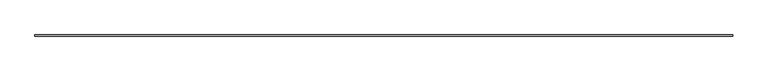
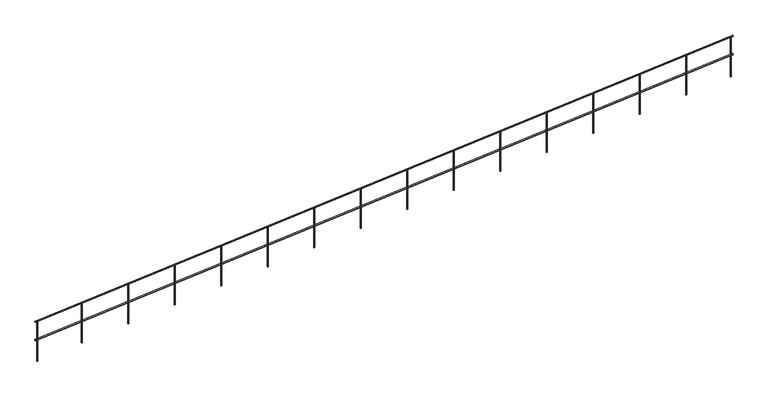
"""IFC4 building model written with IfcOpenShell, lengths in millimetres: railing geometry."""

from ifc_helpers import new_model, si_unit, frame, origin, place, context, project, spatial, ellipse_curve, source, transform, mapped, element, save
from ifc_brep_helpers import plane_surface, cylinder_surface, advanced_brep


def railing_ef706f2a(model_context):
    return source(origin(), model_context, "Body", "AdvancedBrep", [
        advanced_brep(
        [(42716.32048, 67987.0208589, -615.0519932), (42716.32048, 68017.0208589, -615.0519932), (60716.32048, 67987.0208589, 884.9480068), (60716.32048, 68017.0208589, 884.9480068)],
        [
            (0, 1, ellipse_curve(frame((42716.32048, 68002.0208589, -615.0519932), z_axis=(-1.0, 0.0, 0.0), x_axis=(0.0, 0.0, -0.9999999999999999)), 15.0519932, 15.0)),
            (1, 0, ellipse_curve(frame((42716.32048, 68002.0208589, -615.0519932), z_axis=(-1.0, 0.0, 0.0), x_axis=(0.0, 0.0, -0.9999999999999999)), 15.0519932, 15.0)),
            (2, 3, ellipse_curve(frame((60716.32048, 68002.0208589, 884.9480068), z_axis=(1.0, 0.0, 0.0), x_axis=(0.0, 0.0, -0.9999999999999999)), 15.0519932, 15.0)),
            (3, 2, ellipse_curve(frame((60716.32048, 68002.0208589, 884.9480068), z_axis=(1.0, 0.0, 0.0), x_axis=(0.0, 0.0, -0.9999999999999999)), 15.0519932, 15.0)),
            (0, 2),
            (3, 1),
        ],
        [
            plane_surface(frame((42716.32048, 68002.0208589, -600.0), z_axis=(-1.0, 0.0, 0.0), x_axis=(0.0, 1.0, 0.0))),
            plane_surface(frame((60716.32048, 68002.0208589, 900.0), z_axis=(1.0, 0.0, 0.0), x_axis=(0.0, 1.0, 0.0))),
            cylinder_surface(frame((42717.5661622, 68002.0208589, -614.9481864), z_axis=(-0.9965457582448797, 0.0, -0.08304547985373997), x_axis=(0.0, 1.0, 0.0)), 15.0),
        ],
        [
            (0, [[1, 2]]),
            (1, [[3, 4]]),
            (2, [[-1, 5, -4, 6]]),
            (2, [[-2, -6, -3, -5]]),
        ],
    ),
        advanced_brep(
        [(42716.32048, 67987.0208589, -115.0519932), (42716.32048, 68017.0208589, -115.0519932), (60716.32048, 67987.0208589, 1384.9480068), (60716.32048, 68017.0208589, 1384.9480068)],
        [
            (0, 1, ellipse_curve(frame((42716.32048, 68002.0208589, -115.0519932), z_axis=(-1.0, 0.0, 0.0), x_axis=(0.0, 0.0, -0.9999999999999999)), 15.0519932, 15.0)),
            (1, 0, ellipse_curve(frame((42716.32048, 68002.0208589, -115.0519932), z_axis=(-1.0, 0.0, 0.0), x_axis=(0.0, 0.0, -0.9999999999999999)), 15.0519932, 15.0)),
            (2, 3, ellipse_curve(frame((60716.32048, 68002.0208589, 1384.9480068), z_axis=(1.0, 0.0, 0.0), x_axis=(0.0, 0.0, -0.9999999999999999)), 15.0519932, 15.0)),
            (3, 2, ellipse_curve(frame((60716.32048, 68002.0208589, 1384.9480068), z_axis=(1.0, 0.0, 0.0), x_axis=(0.0, 0.0, -0.9999999999999999)), 15.0519932, 15.0)),
            (0, 2),
            (3, 1),
        ],
        [
            plane_surface(frame((42716.32048, 68002.0208589, -100.0), z_axis=(-1.0, 0.0, 0.0), x_axis=(0.0, 1.0, 0.0))),
            plane_surface(frame((60716.32048, 68002.0208589, 1400.0), z_axis=(1.0, 0.0, 0.0), x_axis=(0.0, 1.0, 0.0))),
            cylinder_surface(frame((42717.5661622, 68002.0208589, -114.9481864), z_axis=(-0.9965457582448797, 0.0, -0.08304547985373997), x_axis=(0.0, 1.0, 0.0)), 15.0),
        ],
        [
            (0, [[1, 2]]),
            (1, [[3, 4]]),
            (2, [[-1, 5, -4, 6]]),
            (2, [[-2, -6, -3, -5]]),
        ],
    ),
        advanced_brep(
        [(59516.32048, 68017.0208589, 1269.8960136), (59516.32048, 67987.0208589, 1269.8960136), (59516.32048, 67987.0208589, 200.0), (59516.32048, 68017.0208589, 200.0)],
        [
            (0, 1, ellipse_curve(frame((59516.32048, 68002.0208589, 1269.8960136), z_axis=(0.083045479853741, 0.0, -0.9965457582448796), x_axis=(0.9965457582448797, 0.0, 0.08304547985374044)), 15.0519932, 15.0)),
            (1, 2),
            (2, 3, ellipse_curve(frame((59516.32048, 68002.0208589, 200.0), z_axis=(-0.08304547985373996, 0.0, 0.9965457582448797), x_axis=(0.9965457582448798, 0.0, 0.08304547985373881)), 15.0519932, 15.0)),
            (3, 0),
            (3, 2, ellipse_curve(frame((59516.32048, 68002.0208589, 200.0), z_axis=(-0.08304547985373996, 0.0, 0.9965457582448797), x_axis=(0.9965457582448798, 0.0, 0.08304547985373881)), 15.0519932, 15.0)),
            (1, 0, ellipse_curve(frame((59516.32048, 68002.0208589, 1269.8960136), z_axis=(0.083045479853741, 0.0, -0.9965457582448796), x_axis=(0.9965457582448797, 0.0, 0.08304547985374044)), 15.0519932, 15.0)),
        ],
        [
            cylinder_surface(frame((59516.32048, 68002.0208589, 100.0), z_axis=(0.0, 0.0, 1.0), x_axis=(0.0, -1.0, 0.0)), 15.0),
            plane_surface(frame((59541.32048, 67977.0208589, 1271.9793469), z_axis=(-0.083045479853741, 0.0, 0.9965457582448796), x_axis=(0.0, 1.0, 0.0))),
            plane_surface(frame((59491.32048, 67977.0208589, 197.9166667), z_axis=(0.08304547985373996, 0.0, -0.9965457582448797), x_axis=(0.0, 1.0, 0.0))),
        ],
        [
            (0, [[1, 2, 3, 4]]),
            (0, [[5, -2, 6, -4]]),
            (1, [[-6, -1]]),
            (2, [[-5, -3]]),
        ],
    ),
        advanced_brep(
        [(58316.32048, 68017.0208589, 1169.8960136), (58316.32048, 67987.0208589, 1169.8960136), (58316.32048, 67987.0208589, 100.0), (58316.32048, 68017.0208589, 100.0)],
        [
            (0, 1, ellipse_curve(frame((58316.32048, 68002.0208589, 1169.8960136), z_axis=(0.083045479853741, 0.0, -0.9965457582448796), x_axis=(0.9965457582448797, 0.0, 0.08304547985374044)), 15.0519932, 15.0)),
            (1, 2),
            (2, 3, ellipse_curve(frame((58316.32048, 68002.0208589, 100.0), z_axis=(-0.08304547985373996, 0.0, 0.9965457582448797), x_axis=(0.9965457582448798, 0.0, 0.08304547985373881)), 15.0519932, 15.0)),
            (3, 0),
            (3, 2, ellipse_curve(frame((58316.32048, 68002.0208589, 100.0), z_axis=(-0.08304547985373996, 0.0, 0.9965457582448797), x_axis=(0.9965457582448798, 0.0, 0.08304547985373881)), 15.0519932, 15.0)),
            (1, 0, ellipse_curve(frame((58316.32048, 68002.0208589, 1169.8960136), z_axis=(0.083045479853741, 0.0, -0.9965457582448796), x_axis=(0.9965457582448797, 0.0, 0.08304547985374044)), 15.0519932, 15.0)),
        ],
        [
            cylinder_surface(frame((58316.32048, 68002.0208589, 0.0), z_axis=(0.0, 0.0, 1.0), x_axis=(0.0, -1.0, 0.0)), 15.0),
            plane_surface(frame((58341.32048, 67977.0208589, 1171.9793469), z_axis=(-0.083045479853741, 0.0, 0.9965457582448796), x_axis=(0.0, 1.0, 0.0))),
            plane_surface(frame((58291.32048, 67977.0208589, 97.9166667), z_axis=(0.08304547985373996, 0.0, -0.9965457582448797), x_axis=(0.0, 1.0, 0.0))),
        ],
        [
            (0, [[1, 2, 3, 4]]),
            (0, [[5, -2, 6, -4]]),
            (1, [[-6, -1]]),
            (2, [[-5, -3]]),
        ],
    ),
        advanced_brep(
        [(57116.32048, 68017.0208589, 1069.8960136), (57116.32048, 67987.0208589, 1069.8960136), (57116.32048, 67987.0208589, 0.0), (57116.32048, 68017.0208589, 0.0)],
        [
            (0, 1, ellipse_curve(frame((57116.32048, 68002.0208589, 1069.8960136), z_axis=(0.083045479853741, 0.0, -0.9965457582448796), x_axis=(0.9965457582448797, 0.0, 0.08304547985374044)), 15.0519932, 15.0)),
            (1, 2),
            (2, 3, ellipse_curve(frame((57116.32048, 68002.0208589, 0.0), z_axis=(-0.08304547985373996, 0.0, 0.9965457582448797), x_axis=(0.9965457582448798, 0.0, 0.08304547985373881)), 15.0519932, 15.0)),
            (3, 0),
            (3, 2, ellipse_curve(frame((57116.32048, 68002.0208589, 0.0), z_axis=(-0.08304547985373996, 0.0, 0.9965457582448797), x_axis=(0.9965457582448798, 0.0, 0.08304547985373881)), 15.0519932, 15.0)),
            (1, 0, ellipse_curve(frame((57116.32048, 68002.0208589, 1069.8960136), z_axis=(0.083045479853741, 0.0, -0.9965457582448796), x_axis=(0.9965457582448797, 0.0, 0.08304547985374044)), 15.0519932, 15.0)),
        ],
        [
            cylinder_surface(frame((57116.32048, 68002.0208589, -100.0), z_axis=(0.0, 0.0, 1.0), x_axis=(0.0, -1.0, 0.0)), 15.0),
            plane_surface(frame((57141.32048, 67977.0208589, 1071.9793469), z_axis=(-0.083045479853741, 0.0, 0.9965457582448796), x_axis=(0.0, 1.0, 0.0))),
            plane_surface(frame((57091.32048, 67977.0208589, -2.0833333), z_axis=(0.08304547985373996, 0.0, -0.9965457582448797), x_axis=(0.0, 1.0, 0.0))),
        ],
        [
            (0, [[1, 2, 3, 4]]),
            (0, [[5, -2, 6, -4]]),
            (1, [[-6, -1]]),
            (2, [[-5, -3]]),
        ],
    ),
        advanced_brep(
        [(55916.32048, 68017.0208589, 969.8960136), (55916.32048, 67987.0208589, 969.8960136), (55916.32048, 67987.0208589, -100.0), (55916.32048, 68017.0208589, -100.0)],
        [
            (0, 1, ellipse_curve(frame((55916.32048, 68002.0208589, 969.8960136), z_axis=(0.083045479853741, 0.0, -0.9965457582448796), x_axis=(0.9965457582448797, 0.0, 0.08304547985374044)), 15.0519932, 15.0)),
            (1, 2),
            (2, 3, ellipse_curve(frame((55916.32048, 68002.0208589, -100.0), z_axis=(-0.08304547985373996, 0.0, 0.9965457582448797), x_axis=(0.9965457582448798, 0.0, 0.08304547985373881)), 15.0519932, 15.0)),
            (3, 0),
            (3, 2, ellipse_curve(frame((55916.32048, 68002.0208589, -100.0), z_axis=(-0.08304547985373996, 0.0, 0.9965457582448797), x_axis=(0.9965457582448798, 0.0, 0.08304547985373881)), 15.0519932, 15.0)),
            (1, 0, ellipse_curve(frame((55916.32048, 68002.0208589, 969.8960136), z_axis=(0.083045479853741, 0.0, -0.9965457582448796), x_axis=(0.9965457582448797, 0.0, 0.08304547985374044)), 15.0519932, 15.0)),
        ],
        [
            cylinder_surface(frame((55916.32048, 68002.0208589, -200.0), z_axis=(0.0, 0.0, 1.0), x_axis=(0.0, -1.0, 0.0)), 15.0),
            plane_surface(frame((55941.32048, 67977.0208589, 971.9793469), z_axis=(-0.083045479853741, 0.0, 0.9965457582448796), x_axis=(0.0, 1.0, 0.0))),
            plane_surface(frame((55891.32048, 67977.0208589, -102.0833333), z_axis=(0.08304547985373996, 0.0, -0.9965457582448797), x_axis=(0.0, 1.0, 0.0))),
        ],
        [
            (0, [[1, 2, 3, 4]]),
            (0, [[5, -2, 6, -4]]),
            (1, [[-6, -1]]),
            (2, [[-5, -3]]),
        ],
    ),
        advanced_brep(
        [(54716.32048, 68017.0208589, 869.8960136), (54716.32048, 67987.0208589, 869.8960136), (54716.32048, 67987.0208589, -200.0), (54716.32048, 68017.0208589, -200.0)],
        [
            (0, 1, ellipse_curve(frame((54716.32048, 68002.0208589, 869.8960136), z_axis=(0.083045479853741, 0.0, -0.9965457582448796), x_axis=(0.9965457582448797, 0.0, 0.08304547985374044)), 15.0519932, 15.0)),
            (1, 2),
            (2, 3, ellipse_curve(frame((54716.32048, 68002.0208589, -200.0), z_axis=(-0.08304547985373996, 0.0, 0.9965457582448797), x_axis=(0.9965457582448798, 0.0, 0.08304547985373881)), 15.0519932, 15.0)),
            (3, 0),
            (3, 2, ellipse_curve(frame((54716.32048, 68002.0208589, -200.0), z_axis=(-0.08304547985373996, 0.0, 0.9965457582448797), x_axis=(0.9965457582448798, 0.0, 0.08304547985373881)), 15.0519932, 15.0)),
            (1, 0, ellipse_curve(frame((54716.32048, 68002.0208589, 869.8960136), z_axis=(0.083045479853741, 0.0, -0.9965457582448796), x_axis=(0.9965457582448797, 0.0, 0.08304547985374044)), 15.0519932, 15.0)),
        ],
        [
            cylinder_surface(frame((54716.32048, 68002.0208589, -300.0), z_axis=(0.0, 0.0, 1.0), x_axis=(0.0, -1.0, 0.0)), 15.0),
            plane_surface(frame((54741.32048, 67977.0208589, 871.9793469), z_axis=(-0.083045479853741, 0.0, 0.9965457582448796), x_axis=(0.0, 1.0, 0.0))),
            plane_surface(frame((54691.32048, 67977.0208589, -202.0833333), z_axis=(0.08304547985373996, 0.0, -0.9965457582448797), x_axis=(0.0, 1.0, 0.0))),
        ],
        [
            (0, [[1, 2, 3, 4]]),
            (0, [[5, -2, 6, -4]]),
            (1, [[-6, -1]]),
            (2, [[-5, -3]]),
        ],
    ),
        advanced_brep(
        [(53516.32048, 68017.0208589, 769.8960136), (53516.32048, 67987.0208589, 769.8960136), (53516.32048, 67987.0208589, -300.0), (53516.32048, 68017.0208589, -300.0)],
        [
            (0, 1, ellipse_curve(frame((53516.32048, 68002.0208589, 769.8960136), z_axis=(0.083045479853741, 0.0, -0.9965457582448796), x_axis=(0.9965457582448797, 0.0, 0.08304547985374044)), 15.0519932, 15.0)),
            (1, 2),
            (2, 3, ellipse_curve(frame((53516.32048, 68002.0208589, -300.0), z_axis=(-0.08304547985373996, 0.0, 0.9965457582448797), x_axis=(0.9965457582448798, 0.0, 0.08304547985373881)), 15.0519932, 15.0)),
            (3, 0),
            (3, 2, ellipse_curve(frame((53516.32048, 68002.0208589, -300.0), z_axis=(-0.08304547985373996, 0.0, 0.9965457582448797), x_axis=(0.9965457582448798, 0.0, 0.08304547985373881)), 15.0519932, 15.0)),
            (1, 0, ellipse_curve(frame((53516.32048, 68002.0208589, 769.8960136), z_axis=(0.083045479853741, 0.0, -0.9965457582448796), x_axis=(0.9965457582448797, 0.0, 0.08304547985374044)), 15.0519932, 15.0)),
        ],
        [
            cylinder_surface(frame((53516.32048, 68002.0208589, -400.0), z_axis=(0.0, 0.0, 1.0), x_axis=(0.0, -1.0, 0.0)), 15.0),
            plane_surface(frame((53541.32048, 67977.0208589, 771.9793469), z_axis=(-0.083045479853741, 0.0, 0.9965457582448796), x_axis=(0.0, 1.0, 0.0))),
            plane_surface(frame((53491.32048, 67977.0208589, -302.0833333), z_axis=(0.08304547985373996, 0.0, -0.9965457582448797), x_axis=(0.0, 1.0, 0.0))),
        ],
        [
            (0, [[1, 2, 3, 4]]),
            (0, [[5, -2, 6, -4]]),
            (1, [[-6, -1]]),
            (2, [[-5, -3]]),
        ],
    ),
        advanced_brep(
        [(52316.32048, 68017.0208589, 669.8960136), (52316.32048, 67987.0208589, 669.8960136), (52316.32048, 67987.0208589, -400.0), (52316.32048, 68017.0208589, -400.0)],
        [
            (0, 1, ellipse_curve(frame((52316.32048, 68002.0208589, 669.8960136), z_axis=(0.083045479853741, 0.0, -0.9965457582448796), x_axis=(0.9965457582448797, 0.0, 0.08304547985374044)), 15.0519932, 15.0)),
            (1, 2),
            (2, 3, ellipse_curve(frame((52316.32048, 68002.0208589, -400.0), z_axis=(-0.08304547985373996, 0.0, 0.9965457582448797), x_axis=(0.9965457582448798, 0.0, 0.08304547985373881)), 15.0519932, 15.0)),
            (3, 0),
            (3, 2, ellipse_curve(frame((52316.32048, 68002.0208589, -400.0), z_axis=(-0.08304547985373996, 0.0, 0.9965457582448797), x_axis=(0.9965457582448798, 0.0, 0.08304547985373881)), 15.0519932, 15.0)),
            (1, 0, ellipse_curve(frame((52316.32048, 68002.0208589, 669.8960136), z_axis=(0.083045479853741, 0.0, -0.9965457582448796), x_axis=(0.9965457582448797, 0.0, 0.08304547985374044)), 15.0519932, 15.0)),
        ],
        [
            cylinder_surface(frame((52316.32048, 68002.0208589, -500.0), z_axis=(0.0, 0.0, 1.0), x_axis=(0.0, -1.0, 0.0)), 15.0),
            plane_surface(frame((52341.32048, 67977.0208589, 671.9793469), z_axis=(-0.083045479853741, 0.0, 0.9965457582448796), x_axis=(0.0, 1.0, 0.0))),
            plane_surface(frame((52291.32048, 67977.0208589, -402.0833333), z_axis=(0.08304547985373996, 0.0, -0.9965457582448797), x_axis=(0.0, 1.0, 0.0))),
        ],
        [
            (0, [[1, 2, 3, 4]]),
            (0, [[5, -2, 6, -4]]),
            (1, [[-6, -1]]),
            (2, [[-5, -3]]),
        ],
    ),
        advanced_brep(
        [(51116.32048, 68017.0208589, 569.8960136), (51116.32048, 67987.0208589, 569.8960136), (51116.32048, 67987.0208589, -500.0), (51116.32048, 68017.0208589, -500.0)],
        [
            (0, 1, ellipse_curve(frame((51116.32048, 68002.0208589, 569.8960136), z_axis=(0.083045479853741, 0.0, -0.9965457582448796), x_axis=(0.9965457582448797, 0.0, 0.08304547985374044)), 15.0519932, 15.0)),
            (1, 2),
            (2, 3, ellipse_curve(frame((51116.32048, 68002.0208589, -500.0), z_axis=(-0.08304547985373996, 0.0, 0.9965457582448797), x_axis=(0.9965457582448798, 0.0, 0.08304547985373881)), 15.0519932, 15.0)),
            (3, 0),
            (3, 2, ellipse_curve(frame((51116.32048, 68002.0208589, -500.0), z_axis=(-0.08304547985373996, 0.0, 0.9965457582448797), x_axis=(0.9965457582448798, 0.0, 0.08304547985373881)), 15.0519932, 15.0)),
            (1, 0, ellipse_curve(frame((51116.32048, 68002.0208589, 569.8960136), z_axis=(0.083045479853741, 0.0, -0.9965457582448796), x_axis=(0.9965457582448797, 0.0, 0.08304547985374044)), 15.0519932, 15.0)),
        ],
        [
            cylinder_surface(frame((51116.32048, 68002.0208589, -600.0), z_axis=(0.0, 0.0, 1.0), x_axis=(0.0, -1.0, 0.0)), 15.0),
            plane_surface(frame((51141.32048, 67977.0208589, 571.9793469), z_axis=(-0.083045479853741, 0.0, 0.9965457582448796), x_axis=(0.0, 1.0, 0.0))),
            plane_surface(frame((51091.32048, 67977.0208589, -502.0833333), z_axis=(0.08304547985373996, 0.0, -0.9965457582448797), x_axis=(0.0, 1.0, 0.0))),
        ],
        [
            (0, [[1, 2, 3, 4]]),
            (0, [[5, -2, 6, -4]]),
            (1, [[-6, -1]]),
            (2, [[-5, -3]]),
        ],
    ),
        advanced_brep(
        [(49916.32048, 68017.0208589, 469.8960136), (49916.32048, 67987.0208589, 469.8960136), (49916.32048, 67987.0208589, -600.0), (49916.32048, 68017.0208589, -600.0)],
        [
            (0, 1, ellipse_curve(frame((49916.32048, 68002.0208589, 469.8960136), z_axis=(0.083045479853741, 0.0, -0.9965457582448796), x_axis=(0.9965457582448797, 0.0, 0.08304547985374044)), 15.0519932, 15.0)),
            (1, 2),
            (2, 3, ellipse_curve(frame((49916.32048, 68002.0208589, -600.0), z_axis=(-0.08304547985373996, 0.0, 0.9965457582448797), x_axis=(0.9965457582448798, 0.0, 0.08304547985373881)), 15.0519932, 15.0)),
            (3, 0),
            (3, 2, ellipse_curve(frame((49916.32048, 68002.0208589, -600.0), z_axis=(-0.08304547985373996, 0.0, 0.9965457582448797), x_axis=(0.9965457582448798, 0.0, 0.08304547985373881)), 15.0519932, 15.0)),
            (1, 0, ellipse_curve(frame((49916.32048, 68002.0208589, 469.8960136), z_axis=(0.083045479853741, 0.0, -0.9965457582448796), x_axis=(0.9965457582448797, 0.0, 0.08304547985374044)), 15.0519932, 15.0)),
        ],
        [
            cylinder_surface(frame((49916.32048, 68002.0208589, -700.0), z_axis=(0.0, 0.0, 1.0), x_axis=(0.0, -1.0, 0.0)), 15.0),
            plane_surface(frame((49941.32048, 67977.0208589, 471.9793469), z_axis=(-0.083045479853741, 0.0, 0.9965457582448796), x_axis=(0.0, 1.0, 0.0))),
            plane_surface(frame((49891.32048, 67977.0208589, -602.0833333), z_axis=(0.08304547985373996, 0.0, -0.9965457582448797), x_axis=(0.0, 1.0, 0.0))),
        ],
        [
            (0, [[1, 2, 3, 4]]),
            (0, [[5, -2, 6, -4]]),
            (1, [[-6, -1]]),
            (2, [[-5, -3]]),
        ],
    ),
        advanced_brep(
        [(48716.32048, 68017.0208589, 369.8960136), (48716.32048, 67987.0208589, 369.8960136), (48716.32048, 67987.0208589, -700.0), (48716.32048, 68017.0208589, -700.0)],
        [
            (0, 1, ellipse_curve(frame((48716.32048, 68002.0208589, 369.8960136), z_axis=(0.083045479853741, 0.0, -0.9965457582448796), x_axis=(0.9965457582448797, 0.0, 0.08304547985374044)), 15.0519932, 15.0)),
            (1, 2),
            (2, 3, ellipse_curve(frame((48716.32048, 68002.0208589, -700.0), z_axis=(-0.08304547985373996, 0.0, 0.9965457582448797), x_axis=(0.9965457582448798, 0.0, 0.08304547985373881)), 15.0519932, 15.0)),
            (3, 0),
            (3, 2, ellipse_curve(frame((48716.32048, 68002.0208589, -700.0), z_axis=(-0.08304547985373996, 0.0, 0.9965457582448797), x_axis=(0.9965457582448798, 0.0, 0.08304547985373881)), 15.0519932, 15.0)),
            (1, 0, ellipse_curve(frame((48716.32048, 68002.0208589, 369.8960136), z_axis=(0.083045479853741, 0.0, -0.9965457582448796), x_axis=(0.9965457582448797, 0.0, 0.08304547985374044)), 15.0519932, 15.0)),
        ],
        [
            cylinder_surface(frame((48716.32048, 68002.0208589, -800.0), z_axis=(0.0, 0.0, 1.0), x_axis=(0.0, -1.0, 0.0)), 15.0),
            plane_surface(frame((48741.32048, 67977.0208589, 371.9793469), z_axis=(-0.083045479853741, 0.0, 0.9965457582448796), x_axis=(0.0, 1.0, 0.0))),
            plane_surface(frame((48691.32048, 67977.0208589, -702.0833333), z_axis=(0.08304547985373996, 0.0, -0.9965457582448797), x_axis=(0.0, 1.0, 0.0))),
        ],
        [
            (0, [[1, 2, 3, 4]]),
            (0, [[5, -2, 6, -4]]),
            (1, [[-6, -1]]),
            (2, [[-5, -3]]),
        ],
    ),
        advanced_brep(
        [(47516.32048, 68017.0208589, 269.8960136), (47516.32048, 67987.0208589, 269.8960136), (47516.32048, 67987.0208589, -800.0), (47516.32048, 68017.0208589, -800.0)],
        [
            (0, 1, ellipse_curve(frame((47516.32048, 68002.0208589, 269.8960136), z_axis=(0.083045479853741, 0.0, -0.9965457582448796), x_axis=(0.9965457582448797, 0.0, 0.08304547985374044)), 15.0519932, 15.0)),
            (1, 2),
            (2, 3, ellipse_curve(frame((47516.32048, 68002.0208589, -800.0), z_axis=(-0.08304547985373996, 0.0, 0.9965457582448797), x_axis=(0.9965457582448798, 0.0, 0.08304547985373881)), 15.0519932, 15.0)),
            (3, 0),
            (3, 2, ellipse_curve(frame((47516.32048, 68002.0208589, -800.0), z_axis=(-0.08304547985373996, 0.0, 0.9965457582448797), x_axis=(0.9965457582448798, 0.0, 0.08304547985373881)), 15.0519932, 15.0)),
            (1, 0, ellipse_curve(frame((47516.32048, 68002.0208589, 269.8960136), z_axis=(0.083045479853741, 0.0, -0.9965457582448796), x_axis=(0.9965457582448797, 0.0, 0.08304547985374044)), 15.0519932, 15.0)),
        ],
        [
            cylinder_surface(frame((47516.32048, 68002.0208589, -900.0), z_axis=(0.0, 0.0, 1.0), x_axis=(0.0, -1.0, 0.0)), 15.0),
            plane_surface(frame((47541.32048, 67977.0208589, 271.9793469), z_axis=(-0.083045479853741, 0.0, 0.9965457582448796), x_axis=(0.0, 1.0, 0.0))),
            plane_surface(frame((47491.32048, 67977.0208589, -802.0833333), z_axis=(0.08304547985373996, 0.0, -0.9965457582448797), x_axis=(0.0, 1.0, 0.0))),
        ],
        [
            (0, [[1, 2, 3, 4]]),
            (0, [[5, -2, 6, -4]]),
            (1, [[-6, -1]]),
            (2, [[-5, -3]]),
        ],
    ),
        advanced_brep(
        [(46316.32048, 68017.0208589, 169.8960136), (46316.32048, 67987.0208589, 169.8960136), (46316.32048, 67987.0208589, -900.0), (46316.32048, 68017.0208589, -900.0)],
        [
            (0, 1, ellipse_curve(frame((46316.32048, 68002.0208589, 169.8960136), z_axis=(0.083045479853741, 0.0, -0.9965457582448796), x_axis=(0.9965457582448797, 0.0, 0.08304547985374044)), 15.0519932, 15.0)),
            (1, 2),
            (2, 3, ellipse_curve(frame((46316.32048, 68002.0208589, -900.0), z_axis=(-0.08304547985373996, 0.0, 0.9965457582448797), x_axis=(0.9965457582448798, 0.0, 0.08304547985373881)), 15.0519932, 15.0)),
            (3, 0),
            (3, 2, ellipse_curve(frame((46316.32048, 68002.0208589, -900.0), z_axis=(-0.08304547985373996, 0.0, 0.9965457582448797), x_axis=(0.9965457582448798, 0.0, 0.08304547985373881)), 15.0519932, 15.0)),
            (1, 0, ellipse_curve(frame((46316.32048, 68002.0208589, 169.8960136), z_axis=(0.083045479853741, 0.0, -0.9965457582448796), x_axis=(0.9965457582448797, 0.0, 0.08304547985374044)), 15.0519932, 15.0)),
        ],
        [
            cylinder_surface(frame((46316.32048, 68002.0208589, -1000.0), z_axis=(0.0, 0.0, 1.0), x_axis=(0.0, -1.0, 0.0)), 15.0),
            plane_surface(frame((46341.32048, 67977.0208589, 171.9793469), z_axis=(-0.083045479853741, 0.0, 0.9965457582448796), x_axis=(0.0, 1.0, 0.0))),
            plane_surface(frame((46291.32048, 67977.0208589, -902.0833333), z_axis=(0.08304547985373996, 0.0, -0.9965457582448797), x_axis=(0.0, 1.0, 0.0))),
        ],
        [
            (0, [[1, 2, 3, 4]]),
            (0, [[5, -2, 6, -4]]),
            (1, [[-6, -1]]),
            (2, [[-5, -3]]),
        ],
    ),
        advanced_brep(
        [(45116.32048, 68017.0208589, 69.8960136), (45116.32048, 67987.0208589, 69.8960136), (45116.32048, 67987.0208589, -1000.0), (45116.32048, 68017.0208589, -1000.0)],
        [
            (0, 1, ellipse_curve(frame((45116.32048, 68002.0208589, 69.8960136), z_axis=(0.083045479853741, 0.0, -0.9965457582448796), x_axis=(0.9965457582448797, 0.0, 0.08304547985374044)), 15.0519932, 15.0)),
            (1, 2),
            (2, 3, ellipse_curve(frame((45116.32048, 68002.0208589, -1000.0), z_axis=(-0.08304547985373996, 0.0, 0.9965457582448797), x_axis=(0.9965457582448798, 0.0, 0.08304547985373881)), 15.0519932, 15.0)),
            (3, 0),
            (3, 2, ellipse_curve(frame((45116.32048, 68002.0208589, -1000.0), z_axis=(-0.08304547985373996, 0.0, 0.9965457582448797), x_axis=(0.9965457582448798, 0.0, 0.08304547985373881)), 15.0519932, 15.0)),
            (1, 0, ellipse_curve(frame((45116.32048, 68002.0208589, 69.8960136), z_axis=(0.083045479853741, 0.0, -0.9965457582448796), x_axis=(0.9965457582448797, 0.0, 0.08304547985374044)), 15.0519932, 15.0)),
        ],
        [
            cylinder_surface(frame((45116.32048, 68002.0208589, -1100.0), z_axis=(0.0, 0.0, 1.0), x_axis=(0.0, -1.0, 0.0)), 15.0),
            plane_surface(frame((45141.32048, 67977.0208589, 71.9793469), z_axis=(-0.083045479853741, 0.0, 0.9965457582448796), x_axis=(0.0, 1.0, 0.0))),
            plane_surface(frame((45091.32048, 67977.0208589, -1002.0833333), z_axis=(0.08304547985373996, 0.0, -0.9965457582448797), x_axis=(0.0, 1.0, 0.0))),
        ],
        [
            (0, [[1, 2, 3, 4]]),
            (0, [[5, -2, 6, -4]]),
            (1, [[-6, -1]]),
            (2, [[-5, -3]]),
        ],
    ),
        advanced_brep(
        [(43916.32048, 68017.0208589, -30.1039864), (43916.32048, 67987.0208589, -30.1039864), (43916.32048, 67987.0208589, -1100.0), (43916.32048, 68017.0208589, -1100.0)],
        [
            (0, 1, ellipse_curve(frame((43916.32048, 68002.0208589, -30.1039864), z_axis=(0.083045479853741, 0.0, -0.9965457582448796), x_axis=(0.9965457582448797, 0.0, 0.08304547985374044)), 15.0519932, 15.0)),
            (1, 2),
            (2, 3, ellipse_curve(frame((43916.32048, 68002.0208589, -1100.0), z_axis=(-0.08304547985373996, 0.0, 0.9965457582448797), x_axis=(0.9965457582448798, 0.0, 0.08304547985373881)), 15.0519932, 15.0)),
            (3, 0),
            (3, 2, ellipse_curve(frame((43916.32048, 68002.0208589, -1100.0), z_axis=(-0.08304547985373996, 0.0, 0.9965457582448797), x_axis=(0.9965457582448798, 0.0, 0.08304547985373881)), 15.0519932, 15.0)),
            (1, 0, ellipse_curve(frame((43916.32048, 68002.0208589, -30.1039864), z_axis=(0.083045479853741, 0.0, -0.9965457582448796), x_axis=(0.9965457582448797, 0.0, 0.08304547985374044)), 15.0519932, 15.0)),
        ],
        [
            cylinder_surface(frame((43916.32048, 68002.0208589, -1200.0), z_axis=(0.0, 0.0, 1.0), x_axis=(0.0, -1.0, 0.0)), 15.0),
            plane_surface(frame((43941.32048, 67977.0208589, -28.0206531), z_axis=(-0.083045479853741, 0.0, 0.9965457582448796), x_axis=(0.0, 1.0, 0.0))),
            plane_surface(frame((43891.32048, 67977.0208589, -1102.0833333), z_axis=(0.08304547985373996, 0.0, -0.9965457582448797), x_axis=(0.0, 1.0, 0.0))),
        ],
        [
            (0, [[1, 2, 3, 4]]),
            (0, [[5, -2, 6, -4]]),
            (1, [[-6, -1]]),
            (2, [[-5, -3]]),
        ],
    ),
        advanced_brep(
        [(60666.32048, 68017.0208589, 1365.7293469), (60666.32048, 67987.0208589, 1365.7293469), (60666.32048, 67987.0208589, 295.8333333), (60666.32048, 68017.0208589, 295.8333333)],
        [
            (0, 1, ellipse_curve(frame((60666.32048, 68002.0208589, 1365.7293469), z_axis=(0.083045479853741, 0.0, -0.9965457582448796), x_axis=(0.9965457582448797, 0.0, 0.08304547985374044)), 15.0519932, 15.0)),
            (1, 2),
            (2, 3, ellipse_curve(frame((60666.32048, 68002.0208589, 295.8333333), z_axis=(-0.08304547985373996, 0.0, 0.9965457582448797), x_axis=(0.9965457582448798, 0.0, 0.08304547985373881)), 15.0519932, 15.0)),
            (3, 0),
            (3, 2, ellipse_curve(frame((60666.32048, 68002.0208589, 295.8333333), z_axis=(-0.08304547985373996, 0.0, 0.9965457582448797), x_axis=(0.9965457582448798, 0.0, 0.08304547985373881)), 15.0519932, 15.0)),
            (1, 0, ellipse_curve(frame((60666.32048, 68002.0208589, 1365.7293469), z_axis=(0.083045479853741, 0.0, -0.9965457582448796), x_axis=(0.9965457582448797, 0.0, 0.08304547985374044)), 15.0519932, 15.0)),
        ],
        [
            cylinder_surface(frame((60666.32048, 68002.0208589, 195.8333333), z_axis=(0.0, 0.0, 1.0), x_axis=(0.0, -1.0, 0.0)), 15.0),
            plane_surface(frame((60691.32048, 67977.0208589, 1367.8126802), z_axis=(-0.083045479853741, 0.0, 0.9965457582448796), x_axis=(0.0, 1.0, 0.0))),
            plane_surface(frame((60641.32048, 67977.0208589, 293.75), z_axis=(0.08304547985373996, 0.0, -0.9965457582448797), x_axis=(0.0, 1.0, 0.0))),
        ],
        [
            (0, [[1, 2, 3, 4]]),
            (0, [[5, -2, 6, -4]]),
            (1, [[-6, -1]]),
            (2, [[-5, -3]]),
        ],
    ),
        advanced_brep(
        [(42766.32048, 68017.0208589, -125.9373198), (42766.32048, 67987.0208589, -125.9373198), (42766.32048, 67987.0208589, -1195.8333333), (42766.32048, 68017.0208589, -1195.8333333)],
        [
            (0, 1, ellipse_curve(frame((42766.32048, 68002.0208589, -125.9373198), z_axis=(0.083045479853741, 0.0, -0.9965457582448796), x_axis=(0.9965457582448797, 0.0, 0.08304547985374044)), 15.0519932, 15.0)),
            (1, 2),
            (2, 3, ellipse_curve(frame((42766.32048, 68002.0208589, -1195.8333333), z_axis=(-0.08304547985373996, 0.0, 0.9965457582448797), x_axis=(0.9965457582448798, 0.0, 0.08304547985373881)), 15.0519932, 15.0)),
            (3, 0),
            (3, 2, ellipse_curve(frame((42766.32048, 68002.0208589, -1195.8333333), z_axis=(-0.08304547985373996, 0.0, 0.9965457582448797), x_axis=(0.9965457582448798, 0.0, 0.08304547985373881)), 15.0519932, 15.0)),
            (1, 0, ellipse_curve(frame((42766.32048, 68002.0208589, -125.9373198), z_axis=(0.083045479853741, 0.0, -0.9965457582448796), x_axis=(0.9965457582448797, 0.0, 0.08304547985374044)), 15.0519932, 15.0)),
        ],
        [
            cylinder_surface(frame((42766.32048, 68002.0208589, -1295.8333333), z_axis=(0.0, 0.0, 1.0), x_axis=(0.0, -1.0, 0.0)), 15.0),
            plane_surface(frame((42791.32048, 67977.0208589, -123.8539864), z_axis=(-0.083045479853741, 0.0, 0.9965457582448796), x_axis=(0.0, 1.0, 0.0))),
            plane_surface(frame((42741.32048, 67977.0208589, -1197.9166667), z_axis=(0.08304547985373996, 0.0, -0.9965457582448797), x_axis=(0.0, 1.0, 0.0))),
        ],
        [
            (0, [[1, 2, 3, 4]]),
            (0, [[5, -2, 6, -4]]),
            (1, [[-6, -1]]),
            (2, [[-5, -3]]),
        ],
    ),
    ])


if __name__ == "__main__":
    model = new_model("IFC4")
    model_context = context("Model", 3, world=origin())
    ifc_project = project(units=[si_unit("LENGTHUNIT", "METRE", prefix="MILLI")], contexts=[model_context])
    site = spatial("IfcSite", under=ifc_project)
    building = spatial("IfcBuilding", under=site)
    placement = place(None, origin())
    railing_shape = railing_ef706f2a(model_context)
    element("IfcRailing", 1, at=placement, inside=building, context=model_context, shape_type="MappedRepresentation", body=[
        mapped(railing_shape, transform((0.0, 0.0, 0.0), x_axis=(1.0, 0.0, 0.0), y_axis=(0.0, 1.0, 0.0), z_axis=(0.0, 0.0, 1.0))),
    ])
    save(model, "model.ifc")
